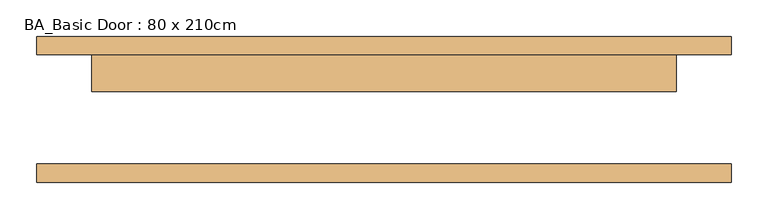
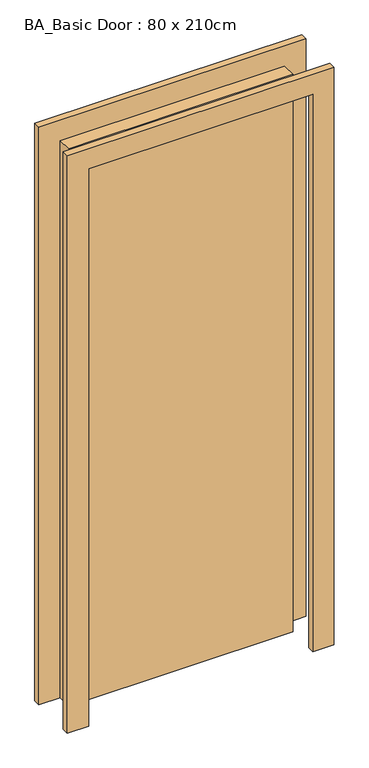
"""IFC4 building model written with IfcOpenShell, lengths in millimetres: door geometry, BA_Basic Door : 80 x 210cm."""

from ifc_helpers import new_model, si_unit, frame, origin, origin_with_axes, place, context, project, spatial, polyline, outline, extrude, source, transform, mapped, element, save


def ba_basic_door_80_x_210cm_4d281df6(model_context):
    return source(origin(), model_context, "Body", "SweptSolid", [
        extrude(outline(polyline([(400.0, 24.0), (-400.0, 24.0), (-400.0, 75.0), (400.0, 75.0), (400.0, 24.0)])), origin_with_axes(), (0.0, 0.0, 1.0), 2100.0),
        extrude(outline(polyline([(2176.0, -476.0), (0.0, -476.0), (0.0, -400.0), (2100.0, -400.0), (2100.0, 400.0), (0.0, 400.0), (0.0, 476.0), (2176.0, 476.0), (2176.0, -476.0)])), frame((0.0, 75.0, 0.0), z_axis=(0.0, 1.0, 0.0), x_axis=(0.0, 0.0, 1.0)), (0.0, 0.0, 1.0), 25.0),
        extrude(outline(polyline([(2176.0, 476.0), (2176.0, -476.0), (0.0, -476.0), (0.0, -400.0), (2100.0, -400.0), (2100.0, 400.0), (0.0, 400.0), (0.0, 476.0), (2176.0, 476.0)])), frame((0.0, -100.0, 0.0), z_axis=(0.0, 1.0, 0.0), x_axis=(0.0, 0.0, 1.0)), (0.0, 0.0, 1.0), 25.0),
    ])


if __name__ == "__main__":
    model = new_model("IFC4")
    model_context = context("Model", 3, world=origin())
    ifc_project = project(units=[si_unit("LENGTHUNIT", "METRE", prefix="MILLI")], contexts=[model_context])
    site = spatial("IfcSite", under=ifc_project)
    building = spatial("IfcBuilding", under=site)
    placement = place(None, origin())
    ba_basic_door_80_x_210cm_shape = ba_basic_door_80_x_210cm_4d281df6(model_context)
    element("IfcDoor", 1, ObjectType="BA_Basic Door : 80 x 210cm", at=placement, inside=building, context=model_context, shape_type="MappedRepresentation", body=[
        mapped(ba_basic_door_80_x_210cm_shape, transform((0.0, 0.0, 0.0), x_axis=(1.0, 0.0, 0.0), y_axis=(0.0, 1.0, 0.0), z_axis=(0.0, 0.0, 1.0))),
    ])
    save(model, "model.ifc")

# Revit data of these elements
# Type "BA_Basic Door : 80 x 210cm"
#   Type Mark = "41"
#   Construction Type Id = "MDOOR"
#   Analytic Construction = "Metal"
#   Window height [instance default] = 1000 mm
#   Thickness = 51 mm
#   Thermal Resistance (R) = 0.270117 (m²·K)/W
#   Cut [instance default] = -100 mm
#   Heat Transfer Coefficient (U) = 3.7021 W/(m²·K)
#   Height = 2100 mm
#   Trim Projection Ext = 25 mm
#   Trim Projection Int = 25 mm
#   Trim Width = 76 mm
#   Width = 800 mm
#   Door window [instance default] = no
#   Define Thermal Properties by = 1
#   Door Material = Default
#   Frame Material = Default
#   Visual Light Transmittance = 0
#   Solar Heat Gain Coefficient = 0
#   Function = (empty or 0)
#   Wall Closure = (empty or 0)
# Element 1 (IfcDoor, "BA_Basic Door : 80 x 210cm")
#   Materials on its faces: "Default"
# Materials
#   "Default": class "Generic", colour RGB 255 255 255, transparency 0, Cost = 0
